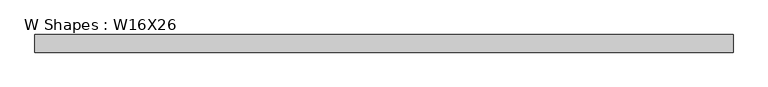
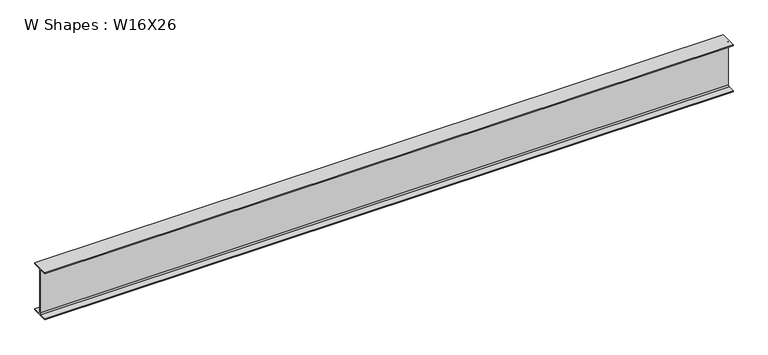
"""IFC4 building model written with IfcOpenShell, lengths in millimetres: beam geometry, W Shapes : W16X26."""

from ifc_helpers import new_model, si_unit, point, frame, frame_2d, origin, place, context, project, spatial, polyline, circle_curve, trimmed, segment, composite_curve, outline, extrude, source, transform, mapped, element, save


def w_shapes_w16x26_29ee5571(model_context):
    return source(origin(), model_context, "Body", "SweptSolid", [
        extrude(outline(composite_curve([segment(polyline([(69.85, -190.627), (69.85, -199.39), (-69.85, -199.39), (-69.85, -190.627), (-13.3858, -190.627)]), True, "CONTINUOUS"), segment(trimmed(circle_curve(frame_2d((-13.3858, -180.4162)), 10.2108), [point((-13.3858, -190.627))], [point((-3.175, -180.4162))], True, "CARTESIAN"), True, "CONTINUOUS"), segment(polyline([(-3.175, -180.4162), (-3.175, 180.4162)]), True, "CONTINUOUS"), segment(trimmed(circle_curve(frame_2d((-13.3858, 180.4162)), 10.2108), [point((-3.175, 180.4162))], [point((-13.3858, 190.627))], True, "CARTESIAN"), True, "CONTINUOUS"), segment(polyline([(-13.3858, 190.627), (-69.85, 190.627), (-69.85, 199.39), (69.85, 199.39), (69.85, 190.627), (13.3858, 190.627)]), True, "CONTINUOUS"), segment(trimmed(circle_curve(frame_2d((13.3858, 180.4162)), 10.2108), [point((13.3858, 190.627))], [point((3.175, 180.4162))], True, "CARTESIAN"), True, "CONTINUOUS"), segment(polyline([(3.175, 180.4162), (3.175, -180.4162)]), True, "CONTINUOUS"), segment(trimmed(circle_curve(frame_2d((13.3858, -180.4162)), 10.2108), [point((3.175, -180.4162))], [point((13.3858, -190.627))], True, "CARTESIAN"), True, "CONTINUOUS"), segment(polyline([(13.3858, -190.627), (69.85, -190.627)]), True, "CONTINUOUS")], self_intersect=False)), frame((-2768.6, 0.0, 0.0), z_axis=(1.0, 0.0, 0.0), x_axis=(0.0, 1.0, 0.0)), (0.0, 0.0, 1.0), 5537.2),
    ])


if __name__ == "__main__":
    model = new_model("IFC4")
    model_context = context("Model", 3, world=origin())
    ifc_project = project(units=[si_unit("LENGTHUNIT", "METRE", prefix="MILLI")], contexts=[model_context])
    site = spatial("IfcSite", under=ifc_project)
    building = spatial("IfcBuilding", under=site)
    placement = place(None, origin())
    w_shapes_w16x26_shape = w_shapes_w16x26_29ee5571(model_context)
    element("IfcBeam", 1, ObjectType="W Shapes : W16X26", at=placement, inside=building, context=model_context, shape_type="MappedRepresentation", body=[
        mapped(w_shapes_w16x26_shape, transform((0.0, 0.0, 0.0), x_axis=(1.0, 0.0, 0.0), y_axis=(0.0, 1.0, 0.0), z_axis=(0.0, 0.0, 1.0))),
    ])
    save(model, "model.ifc")

# Revit data of these elements
# Type "W Shapes : W16X26"
#   Section Name Key = "W16x26"
#   Assembly Code = "B10"
#   Width = 5.500"
#   Web Thickness = 0.250"
#   Web Fillet = 0.402"
#   Warping Constant = 565.00 in⁶
#   Torsional Moment of Inertia = 0.262 in⁴
#   Section Area = 7.68 in²
#   Plastic Modulus weak axis = 5.48 in³
#   Plastic Modulus strong axis = 44.20 in³
#   Perimeter = 4.35 ft²/ft
#   Nominal Weight = 26.00 lbf/ft
#   Moment of Inertia weak axis = 9.59 in⁴
#   Moment of Inertia strong axis = 301.00 in⁴
#   Height = 15.700"
#   Flange Thickness = 0.345"
#   Elastic Modulus weak axis = 3.49 in³
#   Elastic Modulus strong axis = 38.40 in³
#   Centroid Vertical = 7.850"
#   Centroid Horizontal = 2.750"
#   Bolt Spacing = 0' - 3 1/2"
#   Length [instance default] = 5' - 0"
#   Structural Material [instance default] = Steel ASTM A992
#   Principal Axes Angle = 0
# Element 1 (IfcBeam, "W Shapes : W16X26")
#   Structural Material = Steel ASTM A36
#   Materials on its faces: "Steel ASTM A36"
# Materials
#   "Steel ASTM A992": class "Metal", colour RGB 199 199 199, transparency 0, Description = "Structural steel 50ksi", Cost = 0
#   "Steel ASTM A36": class "Metal", colour RGB 199 199 199, transparency 0, Description = "Structural steel, ASTM A36 Grade B, mill finish", Cost = 0
